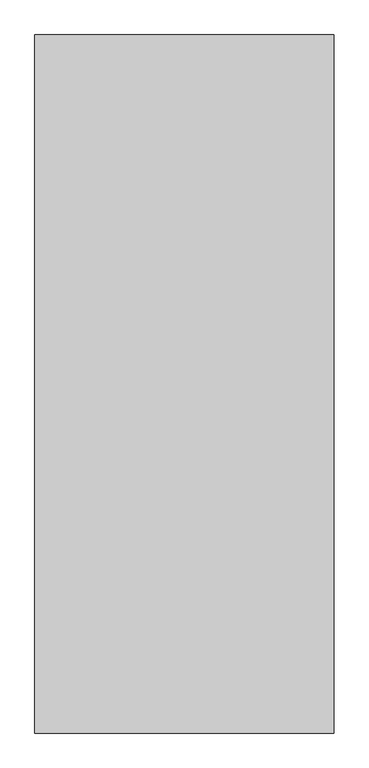
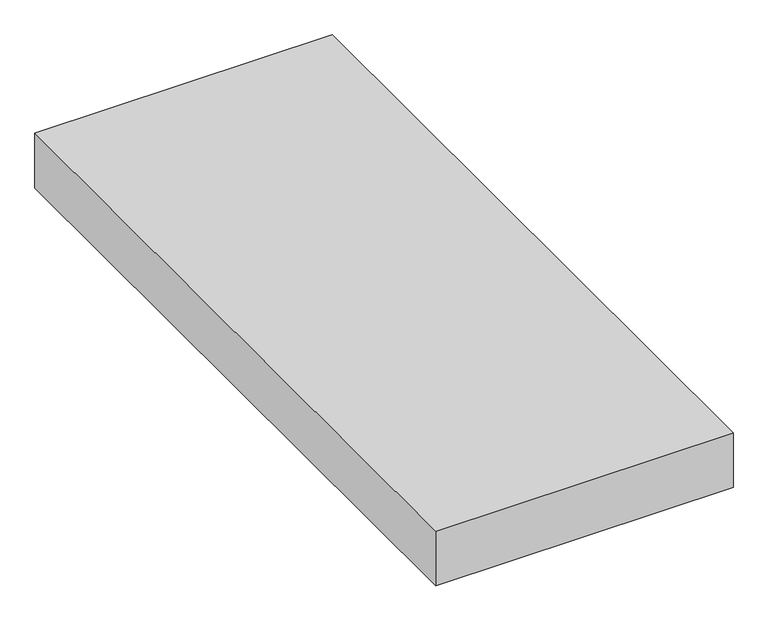
"""IFC4 building model written with IfcOpenShell, lengths in millimetres: proxy geometry, Space Planning Box_hec : Space Planning Box_hec."""

import ifcopenshell
import ifcopenshell.guid

model = None  # the IFC model being written
_history = None  # IfcOwnerHistory: only IFC2X3 demands one
_inside = {}  # id of a spatial element -> (the spatial element, [elements in it])
_under = {}  # id of a project, library or spatial element -> (it, [spatial elements below it])
_declared = {}  # id of a project -> (the project, [libraries it declares])
_typed = {}  # id of a type object -> (the type object, [elements of that type])
_made_of = {}  # id of a material, layer set ... -> (it, [elements and type objects made of it])


def new_model(schema):
    """Start an empty IFC model of exactly this schema.

    Asked for "IFC4X3", IfcOpenShell would pick the latest addendum, in which some entities
    have other attributes; the version numbers below select the first issue.
    IFC2X3 requires an IfcOwnerHistory on every rooted entity: one is made here for all.
    """
    global model, _history
    if schema == "IFC4X3":
        model = ifcopenshell.file(schema_version=(4, 3, 0, 0))
    else:
        model = ifcopenshell.file(schema=schema)
    _inside.clear()
    _under.clear()
    _declared.clear()
    _typed.clear()
    _made_of.clear()
    _history = None
    if model.schema == "IFC2X3":
        org = make("IfcOrganization", Name="unknown")
        user = make(
            "IfcPersonAndOrganization",
            ThePerson=make("IfcPerson", FamilyName="unknown"),
            TheOrganization=org,
        )
        app = make(
            "IfcApplication",
            ApplicationDeveloper=org,
            Version="unknown",
            ApplicationFullName="unknown",
            ApplicationIdentifier="unknown",
        )
        _history = make(
            "IfcOwnerHistory",
            OwningUser=user,
            OwningApplication=app,
            ChangeAction="ADDED",
            CreationDate=0,
        )
    return model


def make(cls, **values):
    """One entity of the class cls with the attributes given. An attribute that is None is left unset."""
    return model.create_entity(
        cls, **{name: value for name, value in values.items() if value is not None}
    )


def rooted(cls, **values):
    """An entity with a GlobalId (a new one), such as an element, a storey or a relation."""
    return make(cls, GlobalId=ifcopenshell.guid.new(), OwnerHistory=_history, **values)


def si_unit(unit_type, name, prefix=None):
    """IfcSIUnit, for example si_unit("LENGTHUNIT", "METRE", prefix="MILLI")."""
    return make("IfcSIUnit", UnitType=unit_type, Prefix=prefix, Name=name)


def assignment(units):
    """IfcUnitAssignment: the units of a project."""
    return None if units is None else make("IfcUnitAssignment", Units=units)


def point(xyz):
    """IfcCartesianPoint."""
    return None if xyz is None else make("IfcCartesianPoint", Coordinates=xyz)


def direction(xyz):
    """IfcDirection."""
    return None if xyz is None else make("IfcDirection", DirectionRatios=xyz)


def frame(location, z_axis=None, x_axis=None):
    """IfcAxis2Placement3D, a coordinate frame: its origin and axes. An axis left out is left unset."""
    return make(
        "IfcAxis2Placement3D",
        Location=point(location),
        Axis=direction(z_axis),
        RefDirection=direction(x_axis),
    )


def origin():
    """The frame at (0, 0, 0) with its axes left unset."""
    return frame((0.0, 0.0, 0.0))


def origin_with_axes():
    """The frame at (0, 0, 0) with the z axis (0, 0, 1) and the x axis (1, 0, 0) written out."""
    return frame((0.0, 0.0, 0.0), z_axis=(0.0, 0.0, 1.0), x_axis=(1.0, 0.0, 0.0))


def place(relative_to, where):
    """IfcLocalPlacement: puts the frame where relative to a parent placement (None: the world)."""
    return make(
        "IfcLocalPlacement", PlacementRelTo=relative_to, RelativePlacement=where
    )


def context(
    kind, dimensions, precision=None, world=None, true_north=None, identifier=None
):
    """IfcGeometricRepresentationContext, for example the 3D "Model" context."""
    return make(
        "IfcGeometricRepresentationContext",
        ContextIdentifier=identifier,
        ContextType=kind,
        CoordinateSpaceDimension=dimensions,
        Precision=precision,
        WorldCoordinateSystem=world,
        TrueNorth=true_north,
    )


def project(units=None, contexts=None):
    """IfcProject with its units and contexts."""
    return rooted(
        "IfcProject",
        Name="project",
        RepresentationContexts=contexts,
        UnitsInContext=assignment(units),
    )


def spatial(cls, under=None, at=None, **own):
    """A site, building, storey or space (cls), placed at a placement, below another one or the project."""
    s = rooted(cls, ObjectPlacement=at, **own)
    if under is not None:
        _under.setdefault(under.id(), (under, []))[1].append(s)
    return s


def polyline(points):
    """IfcPolyline through the points."""
    return make("IfcPolyline", Points=[point(p) for p in points])


def outline(outer, holes=None, kind="AREA"):
    """IfcArbitraryClosedProfileDef: a profile drawn as a closed curve; with holes, ...WithVoids."""
    if holes is None:
        return make("IfcArbitraryClosedProfileDef", ProfileType=kind, OuterCurve=outer)
    return make(
        "IfcArbitraryProfileDefWithVoids",
        ProfileType=kind,
        OuterCurve=outer,
        InnerCurves=holes,
    )


def extrude(swept, where, along, depth):
    """IfcExtrudedAreaSolid: the profile swept, set in the frame where, extruded along a direction by depth."""
    return make(
        "IfcExtrudedAreaSolid",
        SweptArea=swept,
        Position=where,
        ExtrudedDirection=direction(along),
        Depth=depth,
    )


def shape(context_of_items, identifier, shape_type, items):
    """IfcShapeRepresentation: the items that make up one representation, for example the "Body"."""
    return make(
        "IfcShapeRepresentation",
        ContextOfItems=context_of_items,
        RepresentationIdentifier=identifier,
        RepresentationType=shape_type,
        Items=items,
    )


def source(mapping_origin, context_of_items, identifier, shape_type, items):
    """IfcRepresentationMap: a shape defined once, which mapped items show again and again."""
    return make(
        "IfcRepresentationMap",
        MappingOrigin=mapping_origin,
        MappedRepresentation=shape(context_of_items, identifier, shape_type, items),
    )


def transform(
    local_origin,
    x_axis=None,
    y_axis=None,
    z_axis=None,
    scale=None,
    scale2=None,
    scale3=None,
    uniform=True,
):
    """IfcCartesianTransformationOperator3D, or its non-uniform kind. x_axis, y_axis, z_axis: its Axis1, 2, 3."""
    if uniform:
        return make(
            "IfcCartesianTransformationOperator3D",
            Axis1=direction(x_axis),
            Axis2=direction(y_axis),
            LocalOrigin=point(local_origin),
            Scale=scale,
            Axis3=direction(z_axis),
        )
    return make(
        "IfcCartesianTransformationOperator3DnonUniform",
        Axis1=direction(x_axis),
        Axis2=direction(y_axis),
        LocalOrigin=point(local_origin),
        Scale=scale,
        Axis3=direction(z_axis),
        Scale2=scale2,
        Scale3=scale3,
    )


def mapped(mapping_source, mapping_target):
    """IfcMappedItem: shows the shape of a source again, moved by a transform."""
    return make(
        "IfcMappedItem", MappingSource=mapping_source, MappingTarget=mapping_target
    )


def made_of(thing, what):
    """Note that an element or type object is made of a material, layer set ...; save() writes the relation."""
    if what is not None:
        _made_of.setdefault(what.id(), (what, []))[1].append(thing)
    return thing


def element(
    cls,
    number,
    at=None,
    inside=None,
    cuts=None,
    type_object=None,
    material=None,
    context=None,
    identifier="Body",
    shape_type=None,
    held_by="IfcProductDefinitionShape",
    body=None,
    shapes=None,
    **own,
):
    """One element of the class cls, such as IfcWall. Its Tag is "e" and its number.

    at: its placement. inside: the storey or other place that contains it. cuts: it is an
    opening in that element (IfcRelVoidsElement). A single representation is given by context,
    identifier, shape_type and body (its items); several are given by shapes. held_by: the class
    of the entity that holds the representations. save() writes the other relations.
    """
    e = rooted(cls, Tag="e%d" % number, ObjectPlacement=at, **own)
    if body is not None:
        shapes = [shape(context, identifier, shape_type, body)]
    if shapes is not None:
        e.Representation = make(held_by, Representations=shapes)
    if inside is not None:
        _inside.setdefault(inside.id(), (inside, []))[1].append(e)
    if cuts is not None:
        rooted(
            "IfcRelVoidsElement", RelatingBuildingElement=cuts, RelatedOpeningElement=e
        )
    if type_object is not None:
        _typed.setdefault(type_object.id(), (type_object, []))[1].append(e)
    return made_of(e, material)


def aggregate(whole, parts):
    """IfcRelAggregates: a whole, such as a stair, and the parts it consists of."""
    return rooted("IfcRelAggregates", RelatingObject=whole, RelatedObjects=parts)


def save(model, path):
    """Write the relations noted so far, then the file.

    IfcRelAggregates (storeys below a building ...), IfcRelContainedInSpatialStructure (elements
    in a storey), IfcRelDefinesByType, IfcRelAssociatesMaterial and IfcRelDeclares: one each for
    every whole, place, type object, material and project.
    """
    for whole, parts in _under.values():
        aggregate(whole, parts)
    for where, things in _inside.values():
        rooted(
            "IfcRelContainedInSpatialStructure",
            RelatedElements=things,
            RelatingStructure=where,
        )
    for kind, things in _typed.values():
        rooted("IfcRelDefinesByType", RelatedObjects=things, RelatingType=kind)
    for what, things in _made_of.values():
        rooted("IfcRelAssociatesMaterial", RelatedObjects=things, RelatingMaterial=what)
    for by, libraries in _declared.values():
        rooted("IfcRelDeclares", RelatingContext=by, RelatedDefinitions=libraries)
    model.write(path)


def generic_models_bb515c93(model_context):
    return source(origin(), model_context, "Body", "SweptSolid", [
        extrude(outline(polyline([(9000.0, 21000.0), (9000.0, -21000.0), (-9000.0, -21000.0), (-9000.0, 21000.0), (9000.0, 21000.0)])), origin_with_axes(), (0.0, 0.0, 1.0), 3500.0),
    ])


if __name__ == "__main__":
    model = new_model("IFC4")
    model_context = context("Model", 3, world=origin())
    ifc_project = project(units=[si_unit("LENGTHUNIT", "METRE", prefix="MILLI")], contexts=[model_context])
    site = spatial("IfcSite", under=ifc_project)
    building = spatial("IfcBuilding", under=site)
    placement = place(None, origin())
    generic_models_shape = generic_models_bb515c93(model_context)
    element("IfcBuildingElementProxy", 1, Name="Space Planning Box_hec : Space Planning Box_hec", ObjectType="Space Planning Box_hec : Space Planning Box_hec", at=placement, inside=building, context=model_context, shape_type="MappedRepresentation", body=[
        mapped(generic_models_shape, transform((0.0, 0.0, 0.0), x_axis=(1.0, 0.0, 0.0), y_axis=(0.0, 1.0, 0.0), z_axis=(0.0, 0.0, 1.0))),
    ])
    save(model, "model.ifc")

# Revit data of these elements
# Type "Space Planning Box_hec : Space Planning Box_hec"
#   Type Comments = "..."
#   Room Name [instance default] = "?"
#   Interior Finish [instance default] = ""
#   Exterior Finish [instance default] = ""
#   Department [instance default] = ""
#   Assembly Code = "..."
#   ceiling height [instance default] = 0
#   Width [instance default] = 1524 mm
#   Program Area [instance default] = 0.00 m²
#   Length [instance default] = 1524 mm
#   Height [instance default] = 1524 mm
#   Area [instance default] = 2.32258 m²
#   Fill Color [instance default] = Cyan
#   Default Elevation = 0
# Element 1 (IfcBuildingElementProxy, "Space Planning Box_hec : Space Planning Box_hec")
#   Room Name = "Cable Room"
#   Exterior Finish = "N/A..N/A,,EW1..EW2..N/A"
#   Department = "EL"
#   Width = 18000 mm
#   Program Area = 720.00 m²
#   Length = 42000 mm
#   Height = 3500 mm
#   Area = 756.00 m²
#   Fill Color = Orange
#   Materials on its faces: "Orange"
# Materials
#   "Cyan": class "Generic", colour RGB 0 255 255, transparency 0.2, Cost = 0
#   "Orange": class "Generic", colour RGB 255 165 0, transparency 0.2, Cost = 0
